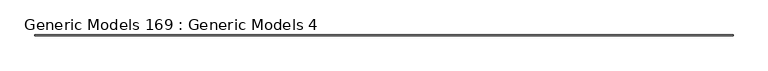
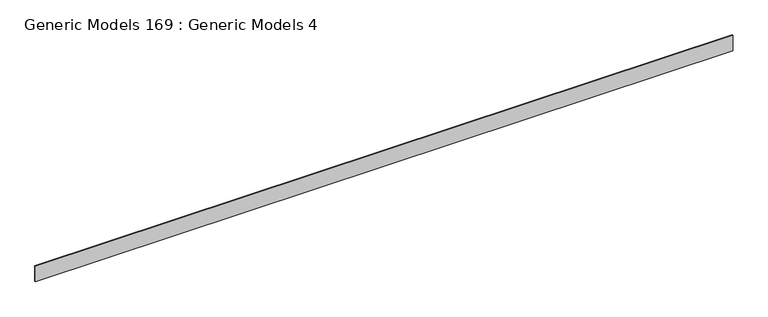
"""IFC4 building model written with IfcOpenShell, lengths in millimetres: proxy geometry, Generic Models 169 : Generic Models 4."""

from ifc_helpers import new_model, si_unit, frame, origin, place, context, project, spatial, polyline, outline, extrude, source, transform, mapped, element, save


def generic_models_169_generic_models_4_bd40d1f0(model_context):
    return source(origin(), model_context, "Body", "SweptSolid", [
        extrude(outline(polyline([(0.0, -15.875), (0.0, 0.0), (12295.7684578, 0.0), (12295.7684578, -15.875), (0.0, -15.875)])), frame((2196.9263704, -5308.6625551, 126783.846), z_axis=(0.0, -1.0913936421275393e-12, 1.0), x_axis=(-1.0, 0.0, 0.0)), (0.0, 0.0, 1.0), 289.0667371),
    ])


if __name__ == "__main__":
    model = new_model("IFC4")
    model_context = context("Model", 3, world=origin())
    ifc_project = project(units=[si_unit("LENGTHUNIT", "METRE", prefix="MILLI")], contexts=[model_context])
    site = spatial("IfcSite", under=ifc_project)
    building = spatial("IfcBuilding", under=site)
    placement = place(None, origin())
    generic_models_169_generic_models_4_shape = generic_models_169_generic_models_4_bd40d1f0(model_context)
    element("IfcBuildingElementProxy", 1, Name="Generic Models 169 : Generic Models 4", ObjectType="Generic Models 169 : Generic Models 4", at=placement, inside=building, context=model_context, shape_type="MappedRepresentation", body=[
        mapped(generic_models_169_generic_models_4_shape, transform((0.0, 0.0, 0.0), x_axis=(1.0, 0.0, 0.0), y_axis=(0.0, 1.0, 0.0), z_axis=(0.0, 0.0, 1.0))),
    ])
    save(model, "model.ifc")

# Revit data of these elements
# Element 1 (IfcBuildingElementProxy, "Generic Models 169 : Generic Models 4")
#   Materials on its faces: "_5/8\" DRYWALL"
# Materials
#   "_5/8\" DRYWALL": class "Generic", colour RGB 191 191 191, transparency 0, Cost = 0
